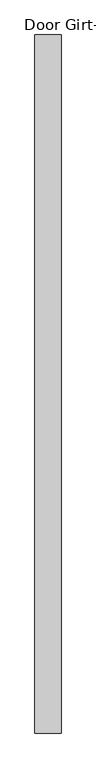
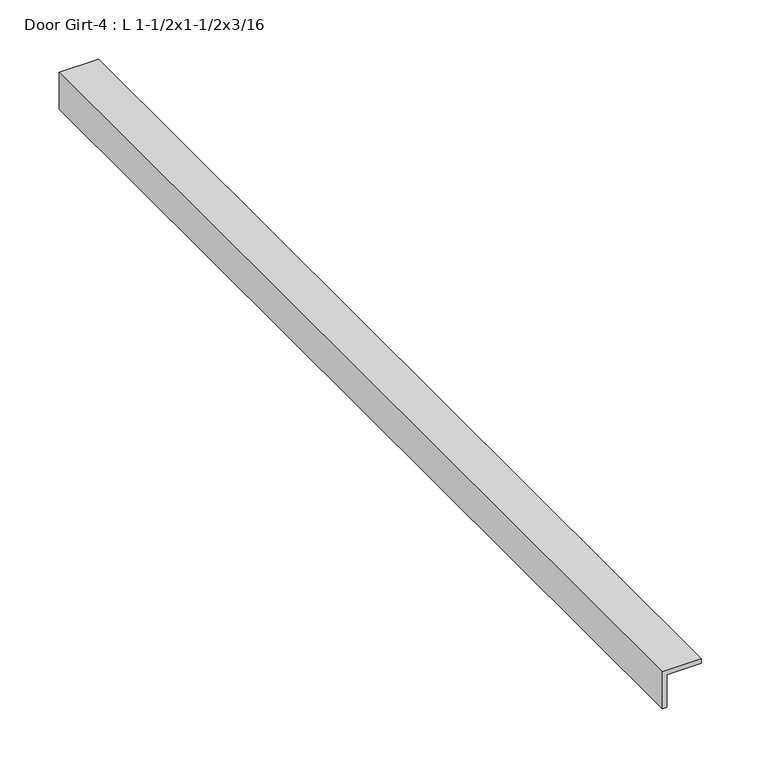
"""IFC4 building model written with IfcOpenShell, lengths in millimetres: proxy geometry, Door Girt-4 : L 1-1/2x1-1/2x3/16."""

import ifcopenshell
import ifcopenshell.guid

model = None  # the IFC model being written
_history = None  # IfcOwnerHistory: only IFC2X3 demands one
_inside = {}  # id of a spatial element -> (the spatial element, [elements in it])
_under = {}  # id of a project, library or spatial element -> (it, [spatial elements below it])
_declared = {}  # id of a project -> (the project, [libraries it declares])
_typed = {}  # id of a type object -> (the type object, [elements of that type])
_made_of = {}  # id of a material, layer set ... -> (it, [elements and type objects made of it])


def new_model(schema):
    """Start an empty IFC model of exactly this schema.

    Asked for "IFC4X3", IfcOpenShell would pick the latest addendum, in which some entities
    have other attributes; the version numbers below select the first issue.
    IFC2X3 requires an IfcOwnerHistory on every rooted entity: one is made here for all.
    """
    global model, _history
    if schema == "IFC4X3":
        model = ifcopenshell.file(schema_version=(4, 3, 0, 0))
    else:
        model = ifcopenshell.file(schema=schema)
    _inside.clear()
    _under.clear()
    _declared.clear()
    _typed.clear()
    _made_of.clear()
    _history = None
    if model.schema == "IFC2X3":
        org = make("IfcOrganization", Name="unknown")
        user = make(
            "IfcPersonAndOrganization",
            ThePerson=make("IfcPerson", FamilyName="unknown"),
            TheOrganization=org,
        )
        app = make(
            "IfcApplication",
            ApplicationDeveloper=org,
            Version="unknown",
            ApplicationFullName="unknown",
            ApplicationIdentifier="unknown",
        )
        _history = make(
            "IfcOwnerHistory",
            OwningUser=user,
            OwningApplication=app,
            ChangeAction="ADDED",
            CreationDate=0,
        )
    return model


def make(cls, **values):
    """One entity of the class cls with the attributes given. An attribute that is None is left unset."""
    return model.create_entity(
        cls, **{name: value for name, value in values.items() if value is not None}
    )


def rooted(cls, **values):
    """An entity with a GlobalId (a new one), such as an element, a storey or a relation."""
    return make(cls, GlobalId=ifcopenshell.guid.new(), OwnerHistory=_history, **values)


def si_unit(unit_type, name, prefix=None):
    """IfcSIUnit, for example si_unit("LENGTHUNIT", "METRE", prefix="MILLI")."""
    return make("IfcSIUnit", UnitType=unit_type, Prefix=prefix, Name=name)


def assignment(units):
    """IfcUnitAssignment: the units of a project."""
    return None if units is None else make("IfcUnitAssignment", Units=units)


def point(xyz):
    """IfcCartesianPoint."""
    return None if xyz is None else make("IfcCartesianPoint", Coordinates=xyz)


def direction(xyz):
    """IfcDirection."""
    return None if xyz is None else make("IfcDirection", DirectionRatios=xyz)


def frame(location, z_axis=None, x_axis=None):
    """IfcAxis2Placement3D, a coordinate frame: its origin and axes. An axis left out is left unset."""
    return make(
        "IfcAxis2Placement3D",
        Location=point(location),
        Axis=direction(z_axis),
        RefDirection=direction(x_axis),
    )


def origin():
    """The frame at (0, 0, 0) with its axes left unset."""
    return frame((0.0, 0.0, 0.0))


def place(relative_to, where):
    """IfcLocalPlacement: puts the frame where relative to a parent placement (None: the world)."""
    return make(
        "IfcLocalPlacement", PlacementRelTo=relative_to, RelativePlacement=where
    )


def context(
    kind, dimensions, precision=None, world=None, true_north=None, identifier=None
):
    """IfcGeometricRepresentationContext, for example the 3D "Model" context."""
    return make(
        "IfcGeometricRepresentationContext",
        ContextIdentifier=identifier,
        ContextType=kind,
        CoordinateSpaceDimension=dimensions,
        Precision=precision,
        WorldCoordinateSystem=world,
        TrueNorth=true_north,
    )


def project(units=None, contexts=None):
    """IfcProject with its units and contexts."""
    return rooted(
        "IfcProject",
        Name="project",
        RepresentationContexts=contexts,
        UnitsInContext=assignment(units),
    )


def spatial(cls, under=None, at=None, **own):
    """A site, building, storey or space (cls), placed at a placement, below another one or the project."""
    s = rooted(cls, ObjectPlacement=at, **own)
    if under is not None:
        _under.setdefault(under.id(), (under, []))[1].append(s)
    return s


def polyline(points):
    """IfcPolyline through the points."""
    return make("IfcPolyline", Points=[point(p) for p in points])


def outline(outer, holes=None, kind="AREA"):
    """IfcArbitraryClosedProfileDef: a profile drawn as a closed curve; with holes, ...WithVoids."""
    if holes is None:
        return make("IfcArbitraryClosedProfileDef", ProfileType=kind, OuterCurve=outer)
    return make(
        "IfcArbitraryProfileDefWithVoids",
        ProfileType=kind,
        OuterCurve=outer,
        InnerCurves=holes,
    )


def extrude(swept, where, along, depth):
    """IfcExtrudedAreaSolid: the profile swept, set in the frame where, extruded along a direction by depth."""
    return make(
        "IfcExtrudedAreaSolid",
        SweptArea=swept,
        Position=where,
        ExtrudedDirection=direction(along),
        Depth=depth,
    )


def shape(context_of_items, identifier, shape_type, items):
    """IfcShapeRepresentation: the items that make up one representation, for example the "Body"."""
    return make(
        "IfcShapeRepresentation",
        ContextOfItems=context_of_items,
        RepresentationIdentifier=identifier,
        RepresentationType=shape_type,
        Items=items,
    )


def source(mapping_origin, context_of_items, identifier, shape_type, items):
    """IfcRepresentationMap: a shape defined once, which mapped items show again and again."""
    return make(
        "IfcRepresentationMap",
        MappingOrigin=mapping_origin,
        MappedRepresentation=shape(context_of_items, identifier, shape_type, items),
    )


def transform(
    local_origin,
    x_axis=None,
    y_axis=None,
    z_axis=None,
    scale=None,
    scale2=None,
    scale3=None,
    uniform=True,
):
    """IfcCartesianTransformationOperator3D, or its non-uniform kind. x_axis, y_axis, z_axis: its Axis1, 2, 3."""
    if uniform:
        return make(
            "IfcCartesianTransformationOperator3D",
            Axis1=direction(x_axis),
            Axis2=direction(y_axis),
            LocalOrigin=point(local_origin),
            Scale=scale,
            Axis3=direction(z_axis),
        )
    return make(
        "IfcCartesianTransformationOperator3DnonUniform",
        Axis1=direction(x_axis),
        Axis2=direction(y_axis),
        LocalOrigin=point(local_origin),
        Scale=scale,
        Axis3=direction(z_axis),
        Scale2=scale2,
        Scale3=scale3,
    )


def mapped(mapping_source, mapping_target):
    """IfcMappedItem: shows the shape of a source again, moved by a transform."""
    return make(
        "IfcMappedItem", MappingSource=mapping_source, MappingTarget=mapping_target
    )


def made_of(thing, what):
    """Note that an element or type object is made of a material, layer set ...; save() writes the relation."""
    if what is not None:
        _made_of.setdefault(what.id(), (what, []))[1].append(thing)
    return thing


def element(
    cls,
    number,
    at=None,
    inside=None,
    cuts=None,
    type_object=None,
    material=None,
    context=None,
    identifier="Body",
    shape_type=None,
    held_by="IfcProductDefinitionShape",
    body=None,
    shapes=None,
    **own,
):
    """One element of the class cls, such as IfcWall. Its Tag is "e" and its number.

    at: its placement. inside: the storey or other place that contains it. cuts: it is an
    opening in that element (IfcRelVoidsElement). A single representation is given by context,
    identifier, shape_type and body (its items); several are given by shapes. held_by: the class
    of the entity that holds the representations. save() writes the other relations.
    """
    e = rooted(cls, Tag="e%d" % number, ObjectPlacement=at, **own)
    if body is not None:
        shapes = [shape(context, identifier, shape_type, body)]
    if shapes is not None:
        e.Representation = make(held_by, Representations=shapes)
    if inside is not None:
        _inside.setdefault(inside.id(), (inside, []))[1].append(e)
    if cuts is not None:
        rooted(
            "IfcRelVoidsElement", RelatingBuildingElement=cuts, RelatedOpeningElement=e
        )
    if type_object is not None:
        _typed.setdefault(type_object.id(), (type_object, []))[1].append(e)
    return made_of(e, material)


def aggregate(whole, parts):
    """IfcRelAggregates: a whole, such as a stair, and the parts it consists of."""
    return rooted("IfcRelAggregates", RelatingObject=whole, RelatedObjects=parts)


def save(model, path):
    """Write the relations noted so far, then the file.

    IfcRelAggregates (storeys below a building ...), IfcRelContainedInSpatialStructure (elements
    in a storey), IfcRelDefinesByType, IfcRelAssociatesMaterial and IfcRelDeclares: one each for
    every whole, place, type object, material and project.
    """
    for whole, parts in _under.values():
        aggregate(whole, parts)
    for where, things in _inside.values():
        rooted(
            "IfcRelContainedInSpatialStructure",
            RelatedElements=things,
            RelatingStructure=where,
        )
    for kind, things in _typed.values():
        rooted("IfcRelDefinesByType", RelatedObjects=things, RelatingType=kind)
    for what, things in _made_of.values():
        rooted("IfcRelAssociatesMaterial", RelatedObjects=things, RelatingMaterial=what)
    for by, libraries in _declared.values():
        rooted("IfcRelDeclares", RelatingContext=by, RelatedDefinitions=libraries)
    model.write(path)


def door_girt_4_l_1_1_2x1_1_2x3_16_602a1831(model_context):
    return source(origin(), model_context, "Body", "SweptSolid", [
        extrude(outline(polyline([(1625.6, 587403.9934739), (1625.6, 587365.8934739), (1587.5, 587365.8934739), (1587.5, 587370.6559739), (1620.8375, 587370.6559739), (1620.8375, 587403.9934739), (1625.6, 587403.9934739)])), frame((0.0, -533937.9163841, 0.0), z_axis=(0.0, 1.0, 0.0), x_axis=(0.0, 0.0, 1.0)), (0.0, 0.0, 1.0), 1016.0),
    ])


if __name__ == "__main__":
    model = new_model("IFC4")
    model_context = context("Model", 3, world=origin())
    ifc_project = project(units=[si_unit("LENGTHUNIT", "METRE", prefix="MILLI")], contexts=[model_context])
    site = spatial("IfcSite", under=ifc_project)
    building = spatial("IfcBuilding", under=site)
    placement = place(None, origin())
    door_girt_4_l_1_1_2x1_1_2x3_16_shape = door_girt_4_l_1_1_2x1_1_2x3_16_602a1831(model_context)
    element("IfcBuildingElementProxy", 1, Name="Door Girt-4 : L 1-1/2x1-1/2x3/16", ObjectType="Door Girt-4 : L 1-1/2x1-1/2x3/16", at=placement, inside=building, context=model_context, shape_type="MappedRepresentation", body=[
        mapped(door_girt_4_l_1_1_2x1_1_2x3_16_shape, transform((0.0, 0.0, 0.0), x_axis=(1.0, 0.0, 0.0), y_axis=(0.0, 1.0, 0.0), z_axis=(0.0, 0.0, 1.0))),
    ])
    save(model, "model.ifc")

# Revit data of these elements
# Element 1 (IfcBuildingElementProxy, "Door Girt-4 : L 1-1/2x1-1/2x3/16")
#   Materials on its faces: "1-1/2\"X1-1/2\" GALV. STL L"
# Materials
#   "1-1/2\"X1-1/2\" GALV. STL L": class "Generic", colour RGB 211 211 207, transparency 0, Cost = 0
